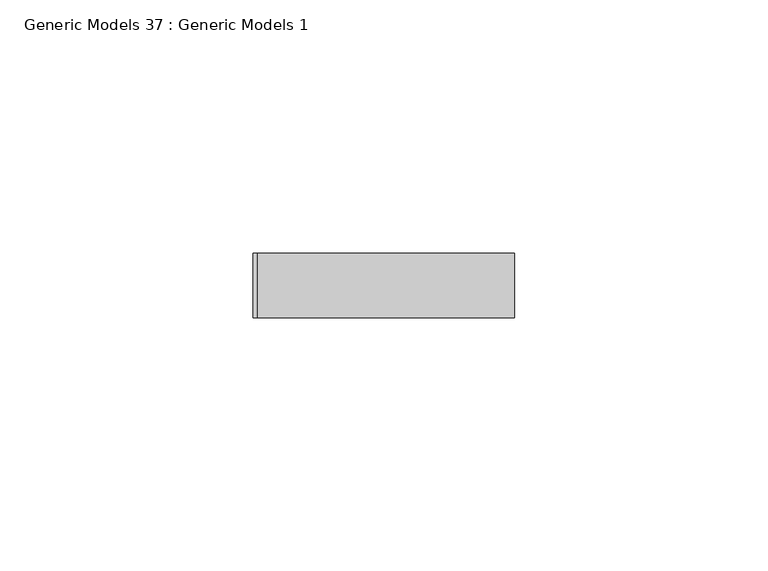
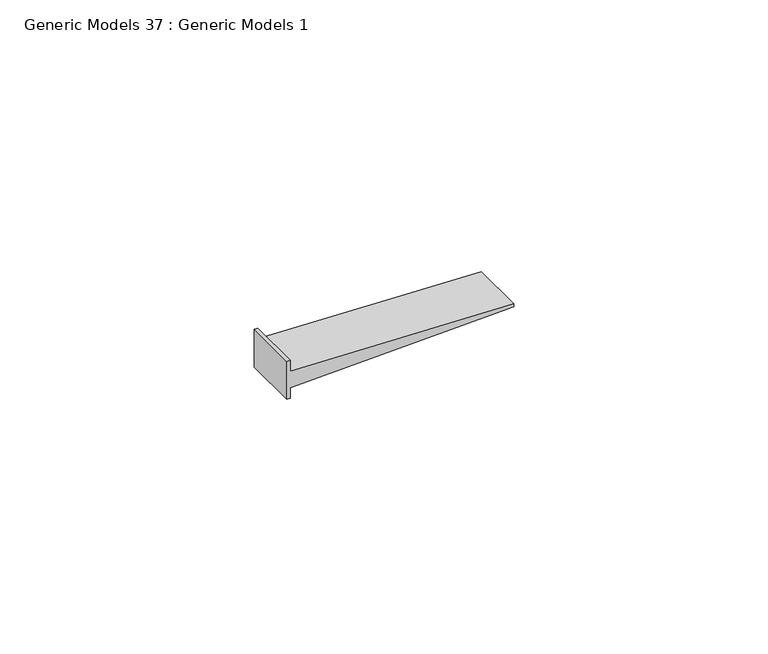
"""IFC4 building model written with IfcOpenShell, lengths in millimetres: proxy geometry, Generic Models 37 : Generic Models 1."""

from ifc_helpers import new_model, si_unit, frame, origin, place, context, project, spatial, polyline, outline, extrude, source, transform, mapped, element, save


def generic_models_37_generic_models_1_916dd7c6(model_context):
    return source(origin(), model_context, "Body", "SweptSolid", [
        extrude(outline(polyline([(2409.6091, 49675.25625), (2400.5159, 49675.25625), (2400.5159, 49676.05), (2403.0657636, 49676.05), (2404.6631527, 49726.85), (2405.4618473, 49726.85), (2407.0592364, 49676.05), (2409.6091, 49676.05), (2409.6091, 49675.25625)])), frame((0.0, 565.15, 0.0), z_axis=(0.0, 1.0, 0.0), x_axis=(0.0, 0.0, 1.0)), (0.0, 0.0, 1.0), 12.7),
    ])


if __name__ == "__main__":
    model = new_model("IFC4")
    model_context = context("Model", 3, world=origin())
    ifc_project = project(units=[si_unit("LENGTHUNIT", "METRE", prefix="MILLI")], contexts=[model_context])
    site = spatial("IfcSite", under=ifc_project)
    building = spatial("IfcBuilding", under=site)
    placement = place(None, origin())
    generic_models_37_generic_models_1_shape = generic_models_37_generic_models_1_916dd7c6(model_context)
    element("IfcBuildingElementProxy", 1, Name="Generic Models 37 : Generic Models 1", ObjectType="Generic Models 37 : Generic Models 1", at=placement, inside=building, context=model_context, shape_type="MappedRepresentation", body=[
        mapped(generic_models_37_generic_models_1_shape, transform((0.0, 0.0, 0.0), x_axis=(1.0, 0.0, 0.0), y_axis=(0.0, 1.0, 0.0), z_axis=(0.0, 0.0, 1.0))),
    ])
    save(model, "model.ifc")

# Revit data of these elements
# Element 1 (IfcBuildingElementProxy, "Generic Models 37 : Generic Models 1")
#   Materials on its faces: "ATTACH GYPSUM BOARD TO STUDS AND NOT TO TOP TRACK"
# Materials
#   "ATTACH GYPSUM BOARD TO STUDS AND NOT TO TOP TRACK": class "Generic", colour RGB 48 48 48, transparency 0, Cost = 0
